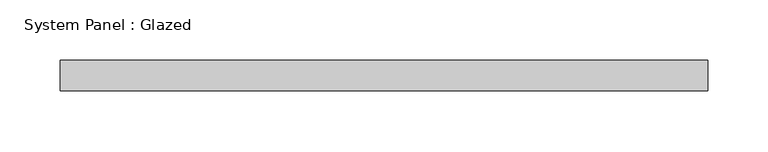
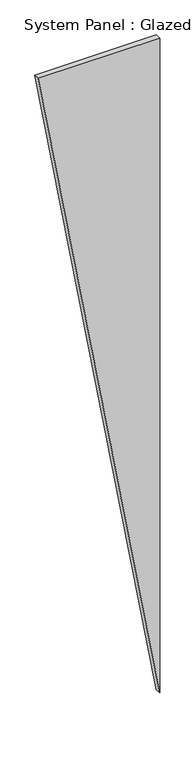
"""IFC4 building model written with IfcOpenShell, lengths in millimetres: plate geometry, System Panel : Glazed."""

import ifcopenshell
import ifcopenshell.guid

model = None  # the IFC model being written
_history = None  # IfcOwnerHistory: only IFC2X3 demands one
_inside = {}  # id of a spatial element -> (the spatial element, [elements in it])
_under = {}  # id of a project, library or spatial element -> (it, [spatial elements below it])
_declared = {}  # id of a project -> (the project, [libraries it declares])
_typed = {}  # id of a type object -> (the type object, [elements of that type])
_made_of = {}  # id of a material, layer set ... -> (it, [elements and type objects made of it])


def new_model(schema):
    """Start an empty IFC model of exactly this schema.

    Asked for "IFC4X3", IfcOpenShell would pick the latest addendum, in which some entities
    have other attributes; the version numbers below select the first issue.
    IFC2X3 requires an IfcOwnerHistory on every rooted entity: one is made here for all.
    """
    global model, _history
    if schema == "IFC4X3":
        model = ifcopenshell.file(schema_version=(4, 3, 0, 0))
    else:
        model = ifcopenshell.file(schema=schema)
    _inside.clear()
    _under.clear()
    _declared.clear()
    _typed.clear()
    _made_of.clear()
    _history = None
    if model.schema == "IFC2X3":
        org = make("IfcOrganization", Name="unknown")
        user = make(
            "IfcPersonAndOrganization",
            ThePerson=make("IfcPerson", FamilyName="unknown"),
            TheOrganization=org,
        )
        app = make(
            "IfcApplication",
            ApplicationDeveloper=org,
            Version="unknown",
            ApplicationFullName="unknown",
            ApplicationIdentifier="unknown",
        )
        _history = make(
            "IfcOwnerHistory",
            OwningUser=user,
            OwningApplication=app,
            ChangeAction="ADDED",
            CreationDate=0,
        )
    return model


def make(cls, **values):
    """One entity of the class cls with the attributes given. An attribute that is None is left unset."""
    return model.create_entity(
        cls, **{name: value for name, value in values.items() if value is not None}
    )


def rooted(cls, **values):
    """An entity with a GlobalId (a new one), such as an element, a storey or a relation."""
    return make(cls, GlobalId=ifcopenshell.guid.new(), OwnerHistory=_history, **values)


def si_unit(unit_type, name, prefix=None):
    """IfcSIUnit, for example si_unit("LENGTHUNIT", "METRE", prefix="MILLI")."""
    return make("IfcSIUnit", UnitType=unit_type, Prefix=prefix, Name=name)


def assignment(units):
    """IfcUnitAssignment: the units of a project."""
    return None if units is None else make("IfcUnitAssignment", Units=units)


def point(xyz):
    """IfcCartesianPoint."""
    return None if xyz is None else make("IfcCartesianPoint", Coordinates=xyz)


def direction(xyz):
    """IfcDirection."""
    return None if xyz is None else make("IfcDirection", DirectionRatios=xyz)


def frame(location, z_axis=None, x_axis=None):
    """IfcAxis2Placement3D, a coordinate frame: its origin and axes. An axis left out is left unset."""
    return make(
        "IfcAxis2Placement3D",
        Location=point(location),
        Axis=direction(z_axis),
        RefDirection=direction(x_axis),
    )


def origin():
    """The frame at (0, 0, 0) with its axes left unset."""
    return frame((0.0, 0.0, 0.0))


def place(relative_to, where):
    """IfcLocalPlacement: puts the frame where relative to a parent placement (None: the world)."""
    return make(
        "IfcLocalPlacement", PlacementRelTo=relative_to, RelativePlacement=where
    )


def context(
    kind, dimensions, precision=None, world=None, true_north=None, identifier=None
):
    """IfcGeometricRepresentationContext, for example the 3D "Model" context."""
    return make(
        "IfcGeometricRepresentationContext",
        ContextIdentifier=identifier,
        ContextType=kind,
        CoordinateSpaceDimension=dimensions,
        Precision=precision,
        WorldCoordinateSystem=world,
        TrueNorth=true_north,
    )


def project(units=None, contexts=None):
    """IfcProject with its units and contexts."""
    return rooted(
        "IfcProject",
        Name="project",
        RepresentationContexts=contexts,
        UnitsInContext=assignment(units),
    )


def spatial(cls, under=None, at=None, **own):
    """A site, building, storey or space (cls), placed at a placement, below another one or the project."""
    s = rooted(cls, ObjectPlacement=at, **own)
    if under is not None:
        _under.setdefault(under.id(), (under, []))[1].append(s)
    return s


def polyline(points):
    """IfcPolyline through the points."""
    return make("IfcPolyline", Points=[point(p) for p in points])


def outline(outer, holes=None, kind="AREA"):
    """IfcArbitraryClosedProfileDef: a profile drawn as a closed curve; with holes, ...WithVoids."""
    if holes is None:
        return make("IfcArbitraryClosedProfileDef", ProfileType=kind, OuterCurve=outer)
    return make(
        "IfcArbitraryProfileDefWithVoids",
        ProfileType=kind,
        OuterCurve=outer,
        InnerCurves=holes,
    )


def extrude(swept, where, along, depth):
    """IfcExtrudedAreaSolid: the profile swept, set in the frame where, extruded along a direction by depth."""
    return make(
        "IfcExtrudedAreaSolid",
        SweptArea=swept,
        Position=where,
        ExtrudedDirection=direction(along),
        Depth=depth,
    )


def shape(context_of_items, identifier, shape_type, items):
    """IfcShapeRepresentation: the items that make up one representation, for example the "Body"."""
    return make(
        "IfcShapeRepresentation",
        ContextOfItems=context_of_items,
        RepresentationIdentifier=identifier,
        RepresentationType=shape_type,
        Items=items,
    )


def source(mapping_origin, context_of_items, identifier, shape_type, items):
    """IfcRepresentationMap: a shape defined once, which mapped items show again and again."""
    return make(
        "IfcRepresentationMap",
        MappingOrigin=mapping_origin,
        MappedRepresentation=shape(context_of_items, identifier, shape_type, items),
    )


def transform(
    local_origin,
    x_axis=None,
    y_axis=None,
    z_axis=None,
    scale=None,
    scale2=None,
    scale3=None,
    uniform=True,
):
    """IfcCartesianTransformationOperator3D, or its non-uniform kind. x_axis, y_axis, z_axis: its Axis1, 2, 3."""
    if uniform:
        return make(
            "IfcCartesianTransformationOperator3D",
            Axis1=direction(x_axis),
            Axis2=direction(y_axis),
            LocalOrigin=point(local_origin),
            Scale=scale,
            Axis3=direction(z_axis),
        )
    return make(
        "IfcCartesianTransformationOperator3DnonUniform",
        Axis1=direction(x_axis),
        Axis2=direction(y_axis),
        LocalOrigin=point(local_origin),
        Scale=scale,
        Axis3=direction(z_axis),
        Scale2=scale2,
        Scale3=scale3,
    )


def mapped(mapping_source, mapping_target):
    """IfcMappedItem: shows the shape of a source again, moved by a transform."""
    return make(
        "IfcMappedItem", MappingSource=mapping_source, MappingTarget=mapping_target
    )


def made_of(thing, what):
    """Note that an element or type object is made of a material, layer set ...; save() writes the relation."""
    if what is not None:
        _made_of.setdefault(what.id(), (what, []))[1].append(thing)
    return thing


def element(
    cls,
    number,
    at=None,
    inside=None,
    cuts=None,
    type_object=None,
    material=None,
    context=None,
    identifier="Body",
    shape_type=None,
    held_by="IfcProductDefinitionShape",
    body=None,
    shapes=None,
    **own,
):
    """One element of the class cls, such as IfcWall. Its Tag is "e" and its number.

    at: its placement. inside: the storey or other place that contains it. cuts: it is an
    opening in that element (IfcRelVoidsElement). A single representation is given by context,
    identifier, shape_type and body (its items); several are given by shapes. held_by: the class
    of the entity that holds the representations. save() writes the other relations.
    """
    e = rooted(cls, Tag="e%d" % number, ObjectPlacement=at, **own)
    if body is not None:
        shapes = [shape(context, identifier, shape_type, body)]
    if shapes is not None:
        e.Representation = make(held_by, Representations=shapes)
    if inside is not None:
        _inside.setdefault(inside.id(), (inside, []))[1].append(e)
    if cuts is not None:
        rooted(
            "IfcRelVoidsElement", RelatingBuildingElement=cuts, RelatedOpeningElement=e
        )
    if type_object is not None:
        _typed.setdefault(type_object.id(), (type_object, []))[1].append(e)
    return made_of(e, material)


def aggregate(whole, parts):
    """IfcRelAggregates: a whole, such as a stair, and the parts it consists of."""
    return rooted("IfcRelAggregates", RelatingObject=whole, RelatedObjects=parts)


def save(model, path):
    """Write the relations noted so far, then the file.

    IfcRelAggregates (storeys below a building ...), IfcRelContainedInSpatialStructure (elements
    in a storey), IfcRelDefinesByType, IfcRelAssociatesMaterial and IfcRelDeclares: one each for
    every whole, place, type object, material and project.
    """
    for whole, parts in _under.values():
        aggregate(whole, parts)
    for where, things in _inside.values():
        rooted(
            "IfcRelContainedInSpatialStructure",
            RelatedElements=things,
            RelatingStructure=where,
        )
    for kind, things in _typed.values():
        rooted("IfcRelDefinesByType", RelatedObjects=things, RelatingType=kind)
    for what, things in _made_of.values():
        rooted("IfcRelAssociatesMaterial", RelatedObjects=things, RelatingMaterial=what)
    for by, libraries in _declared.values():
        rooted("IfcRelDeclares", RelatingContext=by, RelatedDefinitions=libraries)
    model.write(path)


def system_panel_glazed_41c8569a(model_context):
    return source(origin(), model_context, "Body", "SweptSolid", [
        extrude(outline(polyline([(3054.1438606, -268.2393521), (0.0, 268.2393521), (3054.1438606, 268.2393521), (3054.1438606, -268.2393521)])), frame((0.0, -44.45, 0.0), z_axis=(0.0, 1.0, 0.0), x_axis=(0.0, 0.0, 1.0)), (0.0, 0.0, 1.0), 25.4),
    ])


if __name__ == "__main__":
    model = new_model("IFC4")
    model_context = context("Model", 3, world=origin())
    ifc_project = project(units=[si_unit("LENGTHUNIT", "METRE", prefix="MILLI")], contexts=[model_context])
    site = spatial("IfcSite", under=ifc_project)
    building = spatial("IfcBuilding", under=site)
    placement = place(None, origin())
    system_panel_glazed_shape = system_panel_glazed_41c8569a(model_context)
    element("IfcPlate", 1, ObjectType="System Panel : Glazed", at=placement, inside=building, context=model_context, shape_type="MappedRepresentation", body=[
        mapped(system_panel_glazed_shape, transform((0.0, 0.0, 0.0), x_axis=(1.0, 0.0, 0.0), y_axis=(0.0, 1.0, 0.0), z_axis=(0.0, 0.0, 1.0))),
    ])
    save(model, "model.ifc")

# Revit data of these elements
# Type "System Panel : Glazed"
#   Construction Type Id = "GSP4R"
#   Analytic Construction = "1/8 in Pilkington single glazing"
#   Visual Light Transmittance = 0.9
#   Solar Heat Gain Coefficient = 0.86
#   Heat Transfer Coefficient (U) = 1.18115 BTU/(h·ft²·°F)
#   Define Thermal Properties by = 1
# Element 1 (IfcPlate, "System Panel : Glazed")
#   Materials on its faces: "Glass"
# Materials
#   "Glass": class "Glass", colour RGB 0 128 192, transparency 0.75, Description = "Soda Lime Glass", Cost = 0
